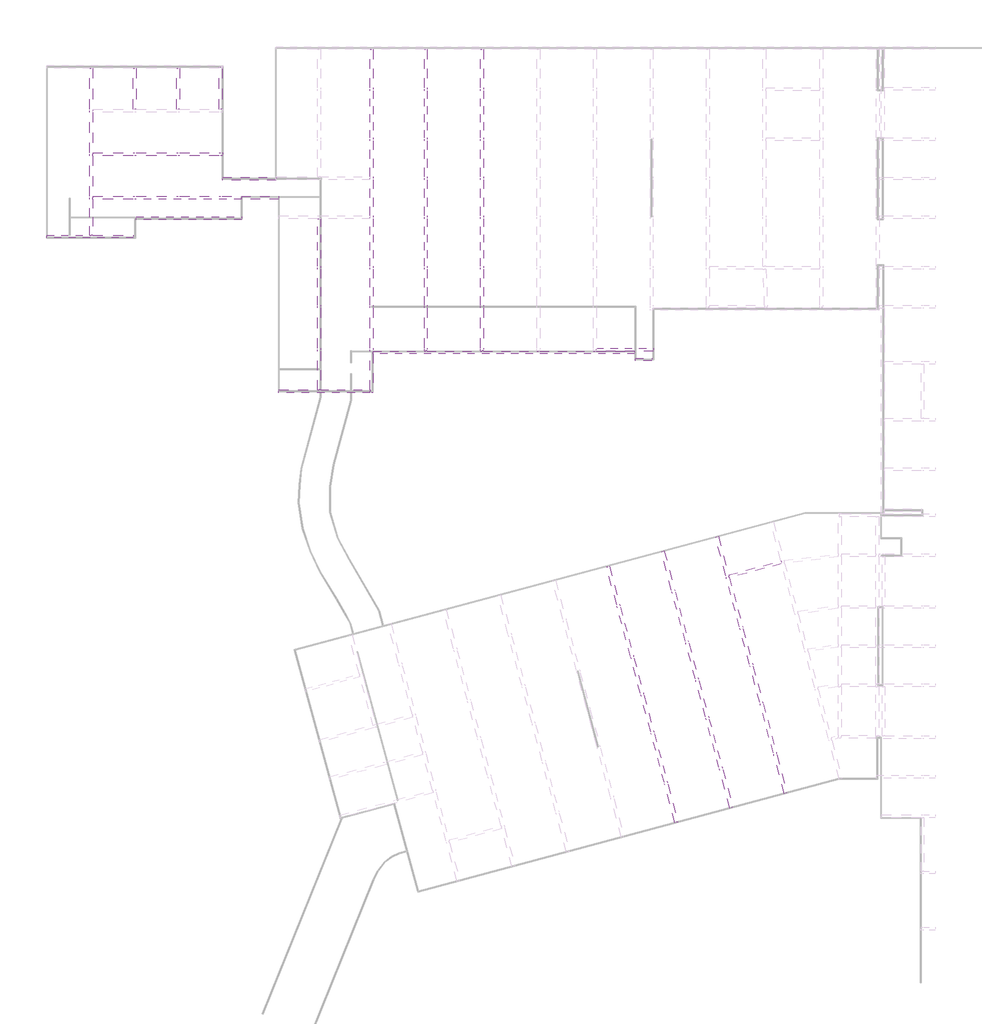
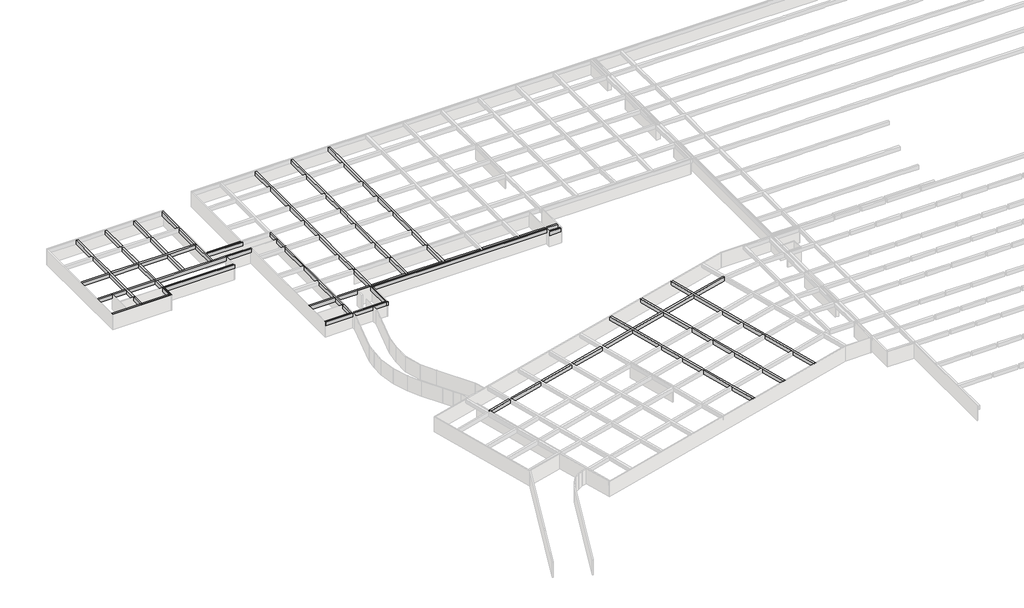
# One storey, part 4 of 14: 22 beams.
# Revit data of these elements (continued)
# Type "混凝土 - 矩形梁 : KL_beam"
#   Length [instance default] = 1524 mm
#   b = 400 mm
#   h = 800 mm
#   Structural Material [instance default] = 混凝土 - 现场浇注混凝土
#   Assembly Code = ""
# Elements 1, 2, 3, 4, 5, 6, 7, 8, 9, 10, 11, 12, 13, 14, 15, 16, 17, 18, 19, 20, 21, 22 (IfcBeam, "混凝土 - 矩形梁 : KL_beam")
#   Comments = ""
#   Structural Material = none
#   Phase Created = 新构造
# Materials
#   "混凝土 - 现场浇注混凝土": class "混凝土", colour RGB 192 192 192, transparency 0
